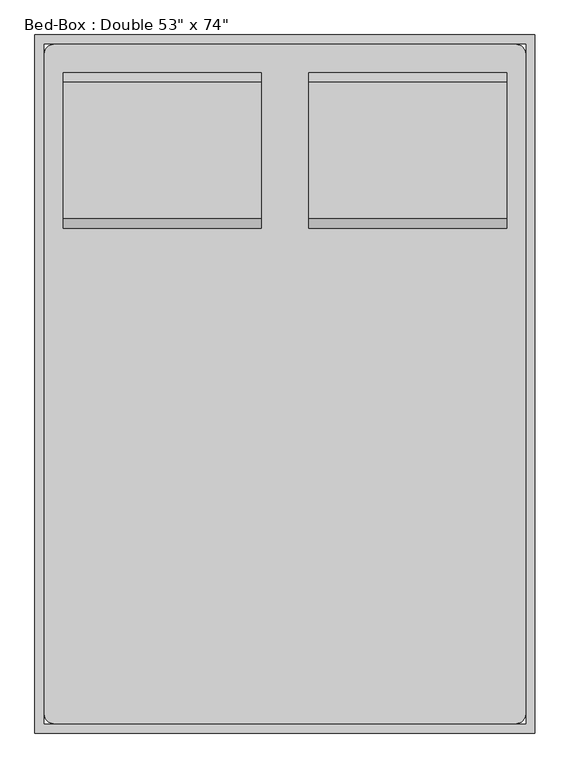
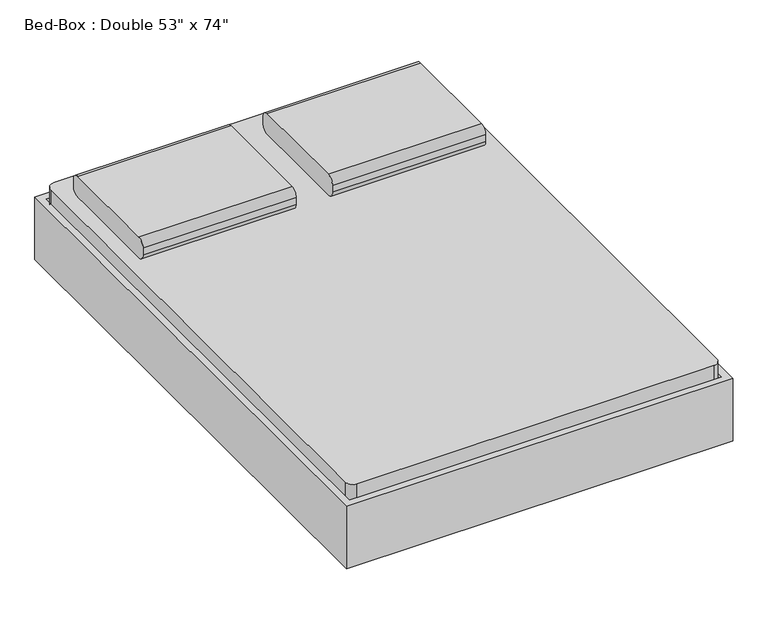
"""IFC4 building model written with IfcOpenShell, lengths in millimetres: furniture geometry."""

import ifcopenshell
import ifcopenshell.guid

model = None  # the IFC model being written
_history = None  # IfcOwnerHistory: only IFC2X3 demands one
_inside = {}  # id of a spatial element -> (the spatial element, [elements in it])
_under = {}  # id of a project, library or spatial element -> (it, [spatial elements below it])
_declared = {}  # id of a project -> (the project, [libraries it declares])
_typed = {}  # id of a type object -> (the type object, [elements of that type])
_made_of = {}  # id of a material, layer set ... -> (it, [elements and type objects made of it])


def new_model(schema):
    """Start an empty IFC model of exactly this schema.

    Asked for "IFC4X3", IfcOpenShell would pick the latest addendum, in which some entities
    have other attributes; the version numbers below select the first issue.
    IFC2X3 requires an IfcOwnerHistory on every rooted entity: one is made here for all.
    """
    global model, _history
    if schema == "IFC4X3":
        model = ifcopenshell.file(schema_version=(4, 3, 0, 0))
    else:
        model = ifcopenshell.file(schema=schema)
    _inside.clear()
    _under.clear()
    _declared.clear()
    _typed.clear()
    _made_of.clear()
    _history = None
    if model.schema == "IFC2X3":
        org = make("IfcOrganization", Name="unknown")
        user = make(
            "IfcPersonAndOrganization",
            ThePerson=make("IfcPerson", FamilyName="unknown"),
            TheOrganization=org,
        )
        app = make(
            "IfcApplication",
            ApplicationDeveloper=org,
            Version="unknown",
            ApplicationFullName="unknown",
            ApplicationIdentifier="unknown",
        )
        _history = make(
            "IfcOwnerHistory",
            OwningUser=user,
            OwningApplication=app,
            ChangeAction="ADDED",
            CreationDate=0,
        )
    return model


def make(cls, **values):
    """One entity of the class cls with the attributes given. An attribute that is None is left unset."""
    return model.create_entity(
        cls, **{name: value for name, value in values.items() if value is not None}
    )


def rooted(cls, **values):
    """An entity with a GlobalId (a new one), such as an element, a storey or a relation."""
    return make(cls, GlobalId=ifcopenshell.guid.new(), OwnerHistory=_history, **values)


def si_unit(unit_type, name, prefix=None):
    """IfcSIUnit, for example si_unit("LENGTHUNIT", "METRE", prefix="MILLI")."""
    return make("IfcSIUnit", UnitType=unit_type, Prefix=prefix, Name=name)


def assignment(units):
    """IfcUnitAssignment: the units of a project."""
    return None if units is None else make("IfcUnitAssignment", Units=units)


def point(xyz):
    """IfcCartesianPoint."""
    return None if xyz is None else make("IfcCartesianPoint", Coordinates=xyz)


def direction(xyz):
    """IfcDirection."""
    return None if xyz is None else make("IfcDirection", DirectionRatios=xyz)


def frame(location, z_axis=None, x_axis=None):
    """IfcAxis2Placement3D, a coordinate frame: its origin and axes. An axis left out is left unset."""
    return make(
        "IfcAxis2Placement3D",
        Location=point(location),
        Axis=direction(z_axis),
        RefDirection=direction(x_axis),
    )


def frame_2d(location, x_axis=None):
    """IfcAxis2Placement2D, a coordinate frame in the plane: its origin and x axis."""
    return make(
        "IfcAxis2Placement2D", Location=point(location), RefDirection=direction(x_axis)
    )


def origin():
    """The frame at (0, 0, 0) with its axes left unset."""
    return frame((0.0, 0.0, 0.0))


def place(relative_to, where):
    """IfcLocalPlacement: puts the frame where relative to a parent placement (None: the world)."""
    return make(
        "IfcLocalPlacement", PlacementRelTo=relative_to, RelativePlacement=where
    )


def context(
    kind, dimensions, precision=None, world=None, true_north=None, identifier=None
):
    """IfcGeometricRepresentationContext, for example the 3D "Model" context."""
    return make(
        "IfcGeometricRepresentationContext",
        ContextIdentifier=identifier,
        ContextType=kind,
        CoordinateSpaceDimension=dimensions,
        Precision=precision,
        WorldCoordinateSystem=world,
        TrueNorth=true_north,
    )


def project(units=None, contexts=None):
    """IfcProject with its units and contexts."""
    return rooted(
        "IfcProject",
        Name="project",
        RepresentationContexts=contexts,
        UnitsInContext=assignment(units),
    )


def spatial(cls, under=None, at=None, **own):
    """A site, building, storey or space (cls), placed at a placement, below another one or the project."""
    s = rooted(cls, ObjectPlacement=at, **own)
    if under is not None:
        _under.setdefault(under.id(), (under, []))[1].append(s)
    return s


def polyline(points):
    """IfcPolyline through the points."""
    return make("IfcPolyline", Points=[point(p) for p in points])


def circle_curve(where, radius):
    """IfcCircle in the frame where."""
    return make("IfcCircle", Position=where, Radius=radius)


def trimmed(basis, trim1, trim2, sense, master):
    """IfcTrimmedCurve: the piece of a basis curve between two trims."""
    return make(
        "IfcTrimmedCurve",
        BasisCurve=basis,
        Trim1=trim1,
        Trim2=trim2,
        SenseAgreement=sense,
        MasterRepresentation=master,
    )


def segment(curve, same_sense, transition):
    """IfcCompositeCurveSegment."""
    return make(
        "IfcCompositeCurveSegment",
        Transition=transition,
        SameSense=same_sense,
        ParentCurve=curve,
    )


def composite_curve(segments, self_intersect=None):
    """IfcCompositeCurve: segments joined end to end."""
    return make("IfcCompositeCurve", Segments=segments, SelfIntersect=self_intersect)


def outline(outer, holes=None, kind="AREA"):
    """IfcArbitraryClosedProfileDef: a profile drawn as a closed curve; with holes, ...WithVoids."""
    if holes is None:
        return make("IfcArbitraryClosedProfileDef", ProfileType=kind, OuterCurve=outer)
    return make(
        "IfcArbitraryProfileDefWithVoids",
        ProfileType=kind,
        OuterCurve=outer,
        InnerCurves=holes,
    )


def extrude(swept, where, along, depth):
    """IfcExtrudedAreaSolid: the profile swept, set in the frame where, extruded along a direction by depth."""
    return make(
        "IfcExtrudedAreaSolid",
        SweptArea=swept,
        Position=where,
        ExtrudedDirection=direction(along),
        Depth=depth,
    )


def shape(context_of_items, identifier, shape_type, items):
    """IfcShapeRepresentation: the items that make up one representation, for example the "Body"."""
    return make(
        "IfcShapeRepresentation",
        ContextOfItems=context_of_items,
        RepresentationIdentifier=identifier,
        RepresentationType=shape_type,
        Items=items,
    )


def source(mapping_origin, context_of_items, identifier, shape_type, items):
    """IfcRepresentationMap: a shape defined once, which mapped items show again and again."""
    return make(
        "IfcRepresentationMap",
        MappingOrigin=mapping_origin,
        MappedRepresentation=shape(context_of_items, identifier, shape_type, items),
    )


def transform(
    local_origin,
    x_axis=None,
    y_axis=None,
    z_axis=None,
    scale=None,
    scale2=None,
    scale3=None,
    uniform=True,
):
    """IfcCartesianTransformationOperator3D, or its non-uniform kind. x_axis, y_axis, z_axis: its Axis1, 2, 3."""
    if uniform:
        return make(
            "IfcCartesianTransformationOperator3D",
            Axis1=direction(x_axis),
            Axis2=direction(y_axis),
            LocalOrigin=point(local_origin),
            Scale=scale,
            Axis3=direction(z_axis),
        )
    return make(
        "IfcCartesianTransformationOperator3DnonUniform",
        Axis1=direction(x_axis),
        Axis2=direction(y_axis),
        LocalOrigin=point(local_origin),
        Scale=scale,
        Axis3=direction(z_axis),
        Scale2=scale2,
        Scale3=scale3,
    )


def mapped(mapping_source, mapping_target):
    """IfcMappedItem: shows the shape of a source again, moved by a transform."""
    return make(
        "IfcMappedItem", MappingSource=mapping_source, MappingTarget=mapping_target
    )


def made_of(thing, what):
    """Note that an element or type object is made of a material, layer set ...; save() writes the relation."""
    if what is not None:
        _made_of.setdefault(what.id(), (what, []))[1].append(thing)
    return thing


def element(
    cls,
    number,
    at=None,
    inside=None,
    cuts=None,
    type_object=None,
    material=None,
    context=None,
    identifier="Body",
    shape_type=None,
    held_by="IfcProductDefinitionShape",
    body=None,
    shapes=None,
    **own,
):
    """One element of the class cls, such as IfcWall. Its Tag is "e" and its number.

    at: its placement. inside: the storey or other place that contains it. cuts: it is an
    opening in that element (IfcRelVoidsElement). A single representation is given by context,
    identifier, shape_type and body (its items); several are given by shapes. held_by: the class
    of the entity that holds the representations. save() writes the other relations.
    """
    e = rooted(cls, Tag="e%d" % number, ObjectPlacement=at, **own)
    if body is not None:
        shapes = [shape(context, identifier, shape_type, body)]
    if shapes is not None:
        e.Representation = make(held_by, Representations=shapes)
    if inside is not None:
        _inside.setdefault(inside.id(), (inside, []))[1].append(e)
    if cuts is not None:
        rooted(
            "IfcRelVoidsElement", RelatingBuildingElement=cuts, RelatedOpeningElement=e
        )
    if type_object is not None:
        _typed.setdefault(type_object.id(), (type_object, []))[1].append(e)
    return made_of(e, material)


def aggregate(whole, parts):
    """IfcRelAggregates: a whole, such as a stair, and the parts it consists of."""
    return rooted("IfcRelAggregates", RelatingObject=whole, RelatedObjects=parts)


def save(model, path):
    """Write the relations noted so far, then the file.

    IfcRelAggregates (storeys below a building ...), IfcRelContainedInSpatialStructure (elements
    in a storey), IfcRelDefinesByType, IfcRelAssociatesMaterial and IfcRelDeclares: one each for
    every whole, place, type object, material and project.
    """
    for whole, parts in _under.values():
        aggregate(whole, parts)
    for where, things in _inside.values():
        rooted(
            "IfcRelContainedInSpatialStructure",
            RelatedElements=things,
            RelatingStructure=where,
        )
    for kind, things in _typed.values():
        rooted("IfcRelDefinesByType", RelatedObjects=things, RelatingType=kind)
    for what, things in _made_of.values():
        rooted("IfcRelAssociatesMaterial", RelatedObjects=things, RelatingMaterial=what)
    for by, libraries in _declared.values():
        rooted("IfcRelDeclares", RelatingContext=by, RelatedDefinitions=libraries)
    model.write(path)


def plane_surface(at):
    """IfcPlane: the flat surface through the origin of the frame at, square to its z axis."""
    return make("IfcPlane", Position=at)


def cylinder_surface(at, radius):
    """IfcCylindricalSurface: all points at the distance radius from the z axis of the frame at."""
    return make("IfcCylindricalSurface", Position=at, Radius=radius)


def revolved_surface(curve, axis_point, axis_direction):
    """IfcSurfaceOfRevolution: the curve turned about the line through axis_point along axis_direction."""
    return make(
        "IfcSurfaceOfRevolution",
        SweptCurve=make("IfcArbitraryOpenProfileDef", ProfileType="CURVE", Curve=curve),
        AxisPosition=make("IfcAxis1Placement", Location=point(axis_point), Axis=direction(axis_direction)),
    )


def advanced_brep(points, edges, surfaces, faces):
    """IfcAdvancedBrep: a solid bounded by faces that lie on surfaces and meet in shared edges.

    An edge is (start, end): straight between two places in points (the first is 0);
    or (start, end, curve); or (start, end, curve, False) where it runs against its curve.
    A face is (place in surfaces, loops), or (place, loops, False) where it looks against
    its surface's normal. A loop lists edges by number (the first is 1), with a minus sign
    where the edge is run from its end to its start. The first loop is the outer one.
    """
    corners = [point(p) for p in points]
    vertices = [make("IfcVertexPoint", VertexGeometry=c) for c in corners]
    made = []
    for start, end, *more in edges:
        made.append(
            make(
                "IfcEdgeCurve",
                EdgeStart=vertices[start],
                EdgeEnd=vertices[end],
                EdgeGeometry=more[0] if more else make("IfcPolyline", Points=[corners[start], corners[end]]),
                SameSense=more[1] if len(more) > 1 else True,
            )
        )
    hull = []
    for where, loops, *sense in faces:
        bounds = []
        for j, loop in enumerate(loops):
            ring = [make("IfcOrientedEdge", EdgeElement=made[abs(k) - 1], Orientation=k > 0) for k in loop]
            bounds.append(
                make(
                    "IfcFaceOuterBound" if j == 0 else "IfcFaceBound",
                    Bound=make("IfcEdgeLoop", EdgeList=ring),
                    Orientation=True,
                )
            )
        hull.append(make("IfcAdvancedFace", Bounds=bounds, FaceSurface=surfaces[where], SameSense=sense[0] if sense else True))
    return make("IfcAdvancedBrep", Outer=make("IfcClosedShell", CfsFaces=hull))


def furniture_bd6c971a(model_context):
    return source(origin(), model_context, "Body", "SolidModel", [
        extrude(outline(composite_curve([segment(polyline([(578.3704918, 406.4), (210.0704918, 406.4)]), True, "CONTINUOUS"), segment(trimmed(circle_curve(frame_2d((210.0704918, 431.8)), 25.4), [point((210.0704918, 406.4))], [point((184.6704918, 431.8))], False, "CARTESIAN"), True, "CONTINUOUS"), segment(polyline([(184.6704918, 431.8), (184.6704918, 457.2)]), True, "CONTINUOUS"), segment(trimmed(circle_curve(frame_2d((210.0704918, 457.2)), 25.4), [point((184.6704918, 457.2))], [point((210.0704918, 482.6))], False, "CARTESIAN"), True, "CONTINUOUS"), segment(polyline([(210.0704918, 482.6), (578.3704918, 482.6)]), True, "CONTINUOUS"), segment(trimmed(circle_curve(frame_2d((578.3704918, 457.2)), 25.4), [point((578.3704918, 482.6))], [point((603.7704918, 457.2))], False, "CARTESIAN"), True, "CONTINUOUS"), segment(polyline([(603.7704918, 457.2), (603.7704918, 431.8)]), True, "CONTINUOUS"), segment(trimmed(circle_curve(frame_2d((578.3704918, 431.8)), 25.4), [point((603.7704918, 431.8))], [point((578.3704918, 406.4))], False, "CARTESIAN"), True, "CONTINUOUS")], self_intersect=False)), frame((402.652459, 0.0, 0.0), z_axis=(1.0, 0.0, 0.0), x_axis=(0.0, 1.0, 0.0)), (0.0, 0.0, 1.0), 533.4),
        extrude(outline(composite_curve([segment(polyline([(578.3704918, 406.4), (210.0704918, 406.4)]), True, "CONTINUOUS"), segment(trimmed(circle_curve(frame_2d((210.0704918, 431.8)), 25.4), [point((210.0704918, 406.4))], [point((184.6704918, 431.8))], False, "CARTESIAN"), True, "CONTINUOUS"), segment(polyline([(184.6704918, 431.8), (184.6704918, 457.2)]), True, "CONTINUOUS"), segment(trimmed(circle_curve(frame_2d((210.0704918, 457.2)), 25.4), [point((184.6704918, 457.2))], [point((210.0704918, 482.6))], False, "CARTESIAN"), True, "CONTINUOUS"), segment(polyline([(210.0704918, 482.6), (578.3704918, 482.6)]), True, "CONTINUOUS"), segment(trimmed(circle_curve(frame_2d((578.3704918, 457.2)), 25.4), [point((578.3704918, 482.6))], [point((603.7704918, 457.2))], False, "CARTESIAN"), True, "CONTINUOUS"), segment(polyline([(603.7704918, 457.2), (603.7704918, 431.8)]), True, "CONTINUOUS"), segment(trimmed(circle_curve(frame_2d((578.3704918, 431.8)), 25.4), [point((603.7704918, 431.8))], [point((578.3704918, 406.4))], False, "CARTESIAN"), True, "CONTINUOUS")], self_intersect=False)), frame((-257.747541, 0.0, 0.0), z_axis=(1.0, 0.0, 0.0), x_axis=(0.0, 1.0, 0.0)), (0.0, 0.0, 1.0), 533.4),
        advanced_brep(
        [(-308.2231784, 451.3704918, 177.8), (-308.2231784, 375.1704918, 177.8), (-308.2231784, 375.1704918, 196.85), (-308.2231784, 451.3704918, 196.85), (-257.4231784, 451.3704918, 177.8), (-257.4231784, 375.1704918, 177.8), (-245.2869899, 375.1704918, 196.85), (-245.2869899, 451.3704918, 196.85), (-181.3523099, 451.3704918, 14.6654962), (-181.3523099, 375.1704918, 14.6654962), (-164.0871466, 375.1704918, 22.716374), (-164.0871466, 451.3704918, 22.716374), (-158.3320921, 375.1704918, 0.0), (-158.3320921, 451.3704918, 0.0), (-158.3320921, 375.1704918, 19.05), (-158.3320921, 451.3704918, 19.05), (-79.7195862, 451.3704918, 0.0), (-79.7195862, 375.1704918, 0.0), (-79.7195862, 375.1704918, 19.05), (-79.7195862, 451.3704918, 19.05), (-67.0195862, 375.1704918, 3.4029547), (-67.0195862, 451.3704918, 3.4029547), (-76.5445862, 375.1704918, 19.9007387), (-76.5445862, 451.3704918, 19.9007387), (-6.922541, 451.3704918, 38.1), (-6.922541, 375.1704918, 38.1), (-12.0269731, 375.1704918, 57.15), (-12.0269731, 451.3704918, 57.15), (685.5518216, 451.3704918, 38.1), (685.5518216, 375.1704918, 38.1), (690.6562537, 375.1704918, 57.15), (690.6562537, 451.3704918, 57.15), (745.6488669, 451.3704918, 3.4029547), (745.6488669, 375.1704918, 3.4029547), (755.1738669, 375.1704918, 19.9007387), (755.1738669, 451.3704918, 19.9007387), (758.3488669, 375.1704918, 0.0), (758.3488669, 451.3704918, 0.0), (758.3488669, 375.1704918, 19.05), (758.3488669, 451.3704918, 19.05), (836.9613728, 451.3704918, 0.0), (836.9613728, 375.1704918, 0.0), (836.9613728, 375.1704918, 19.05), (836.9613728, 451.3704918, 19.05), (859.9815906, 375.1704918, 14.6654962), (859.9815906, 451.3704918, 14.6654962), (842.7164272, 375.1704918, 22.716374), (842.7164272, 451.3704918, 22.716374), (936.052459, 451.3704918, 177.8), (936.052459, 375.1704918, 177.8), (923.9162705, 375.1704918, 196.85), (923.9162705, 451.3704918, 196.85), (986.852459, 451.3704918, 177.8), (986.852459, 451.3704918, 196.85), (986.852459, 375.1704918, 196.85), (986.852459, 375.1704918, 177.8)],
        [
            (0, 1),
            (1, 2),
            (2, 3),
            (3, 0),
            (0, 4),
            (4, 5),
            (5, 1),
            (5, 6),
            (6, 2),
            (6, 7),
            (7, 3),
            (7, 4),
            (4, 8),
            (8, 9),
            (9, 5),
            (9, 10),
            (10, 6),
            (10, 11),
            (11, 7),
            (11, 8),
            (12, 9, circle_curve(frame((-158.3320921, 375.1704918, 25.4), z_axis=(0.0, 1.0, 0.0), x_axis=(-0.9063077870366486, 0.0, -0.42261826174070233)), 25.4)),
            (8, 13, circle_curve(frame((-158.3320921, 451.3704918, 25.4), z_axis=(0.0, -1.0, 0.0), x_axis=(-0.9063077870366486, 0.0, -0.42261826174070233)), 25.4)),
            (13, 12),
            (14, 10, circle_curve(frame((-158.3320921, 375.1704918, 25.4), z_axis=(0.0, 1.0, 0.0), x_axis=(-0.9063077870366486, 0.0, -0.42261826174070233)), 6.35)),
            (12, 14),
            (15, 11, circle_curve(frame((-158.3320921, 451.3704918, 25.4), z_axis=(0.0, 1.0, 0.0), x_axis=(-0.9063077870366486, 0.0, -0.42261826174070233)), 6.35)),
            (14, 15),
            (15, 13),
            (13, 16),
            (16, 17),
            (17, 12),
            (17, 18),
            (18, 14),
            (18, 19),
            (19, 15),
            (19, 16),
            (20, 17, circle_curve(frame((-79.7195862, 375.1704918, 25.4), z_axis=(0.0, 1.0, 0.0), x_axis=(0.0, 0.0, -1.0)), 25.4)),
            (16, 21, circle_curve(frame((-79.7195862, 451.3704918, 25.4), z_axis=(0.0, -1.0, 0.0), x_axis=(0.0, 0.0, -1.0)), 25.4)),
            (21, 20),
            (22, 18, circle_curve(frame((-79.7195862, 375.1704918, 25.4), z_axis=(0.0, 1.0, 0.0), x_axis=(0.0, 0.0, -1.0)), 6.35)),
            (20, 22),
            (23, 19, circle_curve(frame((-79.7195862, 451.3704918, 25.4), z_axis=(0.0, 1.0, 0.0), x_axis=(0.0, 0.0, -1.0)), 6.35)),
            (22, 23),
            (23, 21),
            (21, 24),
            (24, 25),
            (25, 20),
            (25, 26),
            (26, 22),
            (26, 27),
            (27, 23),
            (27, 24),
            (24, 28),
            (28, 29),
            (29, 25),
            (29, 30),
            (30, 26),
            (30, 31),
            (31, 27),
            (31, 28),
            (28, 32),
            (32, 33),
            (33, 29),
            (33, 34),
            (34, 30),
            (34, 35),
            (35, 31),
            (35, 32),
            (36, 33, circle_curve(frame((758.3488669, 375.1704918, 25.4), z_axis=(0.0, 1.0, 0.0), x_axis=(-0.5000000000000463, 0.0, -0.8660254037844118)), 25.4)),
            (32, 37, circle_curve(frame((758.3488669, 451.3704918, 25.4), z_axis=(0.0, -1.0, 0.0), x_axis=(-0.5000000000000463, 0.0, -0.8660254037844118)), 25.4)),
            (37, 36),
            (38, 34, circle_curve(frame((758.3488669, 375.1704918, 25.4), z_axis=(0.0, 1.0, 0.0), x_axis=(-0.5000000000000463, 0.0, -0.8660254037844118)), 6.35)),
            (36, 38),
            (39, 35, circle_curve(frame((758.3488669, 451.3704918, 25.4), z_axis=(0.0, 1.0, 0.0), x_axis=(-0.5000000000000463, 0.0, -0.8660254037844118)), 6.35)),
            (38, 39),
            (39, 37),
            (37, 40),
            (40, 41),
            (41, 36),
            (41, 42),
            (42, 38),
            (42, 43),
            (43, 39),
            (43, 40),
            (44, 41, circle_curve(frame((836.9613728, 375.1704918, 25.4), z_axis=(0.0, 1.0, 0.0), x_axis=(0.0, 0.0, -1.0)), 25.4)),
            (40, 45, circle_curve(frame((836.9613728, 451.3704918, 25.4), z_axis=(0.0, -1.0, 0.0), x_axis=(0.0, 0.0, -1.0)), 25.4)),
            (45, 44),
            (46, 42, circle_curve(frame((836.9613728, 375.1704918, 25.4), z_axis=(0.0, 1.0, 0.0), x_axis=(0.0, 0.0, -1.0)), 6.35)),
            (44, 46),
            (47, 43, circle_curve(frame((836.9613728, 451.3704918, 25.4), z_axis=(0.0, 1.0, 0.0), x_axis=(0.0, 0.0, -1.0)), 6.35)),
            (46, 47),
            (47, 45),
            (45, 48),
            (48, 49),
            (49, 44),
            (49, 50),
            (50, 46),
            (50, 51),
            (51, 47),
            (51, 48),
            (52, 53),
            (53, 54),
            (54, 55),
            (55, 52),
            (48, 52),
            (55, 49),
            (54, 50),
            (53, 51),
        ],
        [
            plane_surface(frame((-308.2231784, 705.3704918, -152.9490627), z_axis=(-1.0, 0.0, 0.0), x_axis=(0.0, 1.0, 0.0))),
            plane_surface(frame((-308.2231784, 451.3704918, 177.8), z_axis=(0.0, 0.0, -1.0), x_axis=(1.0, 0.0, 0.0))),
            plane_surface(frame((-308.2231784, 375.1704918, 177.8), z_axis=(0.0, -1.0, 0.0), x_axis=(1.0, 0.0, 0.0))),
            plane_surface(frame((-308.2231784, 375.1704918, 196.85), z_axis=(0.0, 0.0, 1.0), x_axis=(1.0, 0.0, 0.0))),
            plane_surface(frame((-308.2231784, 451.3704918, 196.85), z_axis=(0.0, 1.0, 0.0), x_axis=(1.0, 0.0, 0.0))),
            plane_surface(frame((-257.4231784, 451.3704918, 177.8), z_axis=(-0.9063077870366488, 0.0, -0.42261826174070194), x_axis=(0.42261826174070194, 0.0, -0.9063077870366488))),
            plane_surface(frame((-257.4231784, 375.1704918, 177.8), z_axis=(0.0, -1.0, 0.0), x_axis=(0.42261826174070194, 0.0, -0.9063077870366488))),
            plane_surface(frame((-245.2869899, 375.1704918, 196.85), z_axis=(0.9063077870366487, 0.0, 0.4226182617407021), x_axis=(0.4226182617407021, 0.0, -0.9063077870366487))),
            plane_surface(frame((-245.2869899, 451.3704918, 196.85), z_axis=(0.0, 1.0, 0.0), x_axis=(0.4226182617407021, 0.0, -0.9063077870366487))),
            cylinder_surface(frame((-158.3320921, 705.3704918, 25.4), z_axis=(0.0, -1.0, 0.0), x_axis=(-0.9063077870366486, 0.0, -0.42261826174070233)), 25.4),
            plane_surface(frame((-158.3320921, 375.1704918, 25.4), z_axis=(0.0, -1.0, 0.0), x_axis=(-0.9063077870366486, 0.0, -0.42261826174070233))),
            revolved_surface(polyline([(-164.08714654768272, 375.1704918, 22.71637403794654), (-164.08714654768272, 451.3704918, 22.71637403794654)]), (-158.3320921, 705.3704918, 25.4), (0.0, -1.0, 0.0)),
            plane_surface(frame((-158.3320921, 451.3704918, 25.4), z_axis=(0.0, 1.0, 0.0), x_axis=(-0.9063077870366486, 0.0, -0.42261826174070233))),
            plane_surface(frame((-158.3320921, 451.3704918, 0.0), z_axis=(0.0, 0.0, -1.0), x_axis=(1.0, 0.0, 0.0))),
            plane_surface(frame((-158.3320921, 375.1704918, 0.0), z_axis=(0.0, -1.0, 0.0), x_axis=(1.0, 0.0, 0.0))),
            plane_surface(frame((-158.3320921, 375.1704918, 19.05), z_axis=(0.0, 0.0, 1.0), x_axis=(1.0, 0.0, 0.0))),
            plane_surface(frame((-158.3320921, 451.3704918, 19.05), z_axis=(0.0, 1.0, 0.0), x_axis=(1.0, 0.0, 0.0))),
            cylinder_surface(frame((-79.7195862, 705.3704918, 25.4), z_axis=(0.0, -1.0, 0.0), x_axis=(0.0, 0.0, -1.0)), 25.4),
            plane_surface(frame((-79.7195862, 375.1704918, 25.4), z_axis=(0.0, -1.0, 0.0), x_axis=(0.0, 0.0, -1.0))),
            revolved_surface(polyline([(-79.7195862, 375.1704918, 19.049999999999997), (-79.7195862, 451.3704918, 19.049999999999997)]), (-79.7195862, 705.3704918, 25.4), (0.0, -1.0, 0.0)),
            plane_surface(frame((-79.7195862, 451.3704918, 25.4), z_axis=(0.0, 1.0, 0.0), x_axis=(0.0, 0.0, -1.0))),
            plane_surface(frame((-67.0195862, 451.3704918, 3.4029547), z_axis=(0.4999999999998774, 0.0, -0.8660254037845095), x_axis=(0.8660254037845095, 0.0, 0.4999999999998774))),
            plane_surface(frame((-67.0195862, 375.1704918, 3.4029547), z_axis=(0.0, -1.0, 0.0), x_axis=(0.866025403784509, 0.0, 0.49999999999987815))),
            plane_surface(frame((-76.5445862, 375.1704918, 19.9007387), z_axis=(-0.49999999999987754, 0.0, 0.8660254037845093), x_axis=(0.8660254037845093, 0.0, 0.49999999999987754))),
            plane_surface(frame((-76.5445862, 451.3704918, 19.9007387), z_axis=(0.0, 1.0000000000000002, 0.0), x_axis=(0.8660254037845091, 0.0, 0.49999999999987815))),
            plane_surface(frame((-6.922541, 451.3704918, 38.1), z_axis=(0.0, 0.0, -1.0), x_axis=(1.0, 0.0, 0.0))),
            plane_surface(frame((-6.922541, 375.1704918, 38.1), z_axis=(0.0, -1.0, 0.0), x_axis=(1.0, 0.0, 0.0))),
            plane_surface(frame((-12.0269731, 375.1704918, 57.15), z_axis=(0.0, 0.0, 1.0), x_axis=(1.0, 0.0, 0.0))),
            plane_surface(frame((-12.0269731, 451.3704918, 57.15), z_axis=(0.0, 1.0, 0.0), x_axis=(1.0, 0.0, 0.0))),
            plane_surface(frame((685.5518216, 451.3704918, 38.1), z_axis=(-0.500000000000047, 0.0, -0.8660254037844115), x_axis=(0.8660254037844115, 0.0, -0.500000000000047))),
            plane_surface(frame((685.5518216, 375.1704918, 38.1), z_axis=(0.0, -1.0, 0.0), x_axis=(0.8660254037844116, 0.0, -0.500000000000047))),
            plane_surface(frame((690.6562537, 375.1704918, 57.15), z_axis=(0.5000000000000456, 0.0, 0.8660254037844124), x_axis=(0.8660254037844124, 0.0, -0.5000000000000456))),
            plane_surface(frame((690.6562537, 451.3704918, 57.15), z_axis=(0.0, 1.0, 0.0), x_axis=(0.8660254037844124, 0.0, -0.5000000000000456))),
            cylinder_surface(frame((758.3488669, 705.3704918, 25.4), z_axis=(0.0, -1.0, 0.0), x_axis=(-0.5000000000000463, 0.0, -0.8660254037844118)), 25.4),
            plane_surface(frame((758.3488669, 375.1704918, 25.4), z_axis=(0.0, -1.0000000000000002, 0.0), x_axis=(-0.5000000000000464, 0.0, -0.866025403784412))),
            revolved_surface(polyline([(755.1738668999997, 375.1704918, 19.90073868596898), (755.1738668999997, 451.3704918, 19.90073868596898)]), (758.3488669, 705.3704918, 25.4), (0.0, -1.0, 0.0)),
            plane_surface(frame((758.3488669, 451.3704918, 25.4), z_axis=(0.0, 1.0000000000000002, 0.0), x_axis=(-0.5000000000000464, 0.0, -0.866025403784412))),
            plane_surface(frame((758.3488669, 451.3704918, 0.0), z_axis=(0.0, 0.0, -1.0), x_axis=(1.0, 0.0, 0.0))),
            plane_surface(frame((758.3488669, 375.1704918, 0.0), z_axis=(0.0, -1.0, 0.0), x_axis=(1.0, 0.0, 0.0))),
            plane_surface(frame((758.3488669, 375.1704918, 19.05), z_axis=(0.0, 0.0, 1.0), x_axis=(1.0, 0.0, 0.0))),
            plane_surface(frame((758.3488669, 451.3704918, 19.05), z_axis=(0.0, 1.0, 0.0), x_axis=(1.0, 0.0, 0.0))),
            cylinder_surface(frame((836.9613728, 705.3704918, 25.4), z_axis=(0.0, -1.0, 0.0), x_axis=(0.0, 0.0, -1.0)), 25.4),
            plane_surface(frame((836.9613728, 375.1704918, 25.4), z_axis=(0.0, -1.0, 0.0), x_axis=(0.0, 0.0, -1.0))),
            revolved_surface(polyline([(836.9613728, 375.1704918, 19.049999999999997), (836.9613728, 451.3704918, 19.049999999999997)]), (836.9613728, 705.3704918, 25.4), (0.0, -1.0, 0.0)),
            plane_surface(frame((836.9613728, 451.3704918, 25.4), z_axis=(0.0, 1.0, 0.0), x_axis=(0.0, 0.0, -1.0))),
            plane_surface(frame((859.9815906, 451.3704918, 14.6654962), z_axis=(0.9063077870366798, 0.0, -0.4226182617406355), x_axis=(0.4226182617406355, 0.0, 0.9063077870366798))),
            plane_surface(frame((859.9815906, 375.1704918, 14.6654962), z_axis=(0.0, -1.0, 0.0), x_axis=(0.4226182617406356, 0.0, 0.9063077870366797))),
            plane_surface(frame((842.7164272, 375.1704918, 22.716374), z_axis=(-0.9063077870366797, 0.0, 0.4226182617406358), x_axis=(0.4226182617406358, 0.0, 0.9063077870366797))),
            plane_surface(frame((842.7164272, 451.3704918, 22.716374), z_axis=(0.0, 1.0000000000000002, 0.0), x_axis=(0.42261826174063544, 0.0, 0.9063077870366799))),
            plane_surface(frame((986.852459, 705.3704918, -152.9490627), z_axis=(1.0, 0.0, 0.0), x_axis=(0.0, 1.0, 0.0))),
            plane_surface(frame((936.052459, 451.3704918, 177.8), z_axis=(0.0, 0.0, -1.0), x_axis=(1.0, 0.0, 0.0))),
            plane_surface(frame((936.052459, 375.1704918, 177.8), z_axis=(0.0, -1.0, 0.0), x_axis=(1.0, 0.0, 0.0))),
            plane_surface(frame((923.9162705, 375.1704918, 196.85), z_axis=(0.0, 0.0, 1.0), x_axis=(1.0, 0.0, 0.0))),
            plane_surface(frame((923.9162705, 451.3704918, 196.85), z_axis=(0.0, 1.0, 0.0), x_axis=(1.0, 0.0, 0.0))),
        ],
        [
            (0, [[1, 2, 3, 4]]),
            (1, [[-1, 5, 6, 7]]),
            (2, [[-2, -7, 8, 9]]),
            (3, [[-3, -9, 10, 11]]),
            (4, [[-4, -11, 12, -5]]),
            (5, [[-6, 13, 14, 15]]),
            (6, [[-8, -15, 16, 17]]),
            (7, [[-10, -17, 18, 19]]),
            (8, [[-12, -19, 20, -13]]),
            (9, [[21, -14, 22, 23]]),
            (10, [[24, -16, -21, 25]]),
            (11, [[26, -18, -24, 27]]),
            (12, [[-22, -20, -26, 28]]),
            (13, [[-23, 29, 30, 31]]),
            (14, [[-25, -31, 32, 33]]),
            (15, [[-27, -33, 34, 35]]),
            (16, [[-28, -35, 36, -29]]),
            (17, [[37, -30, 38, 39]]),
            (18, [[40, -32, -37, 41]]),
            (19, [[42, -34, -40, 43]]),
            (20, [[-38, -36, -42, 44]]),
            (21, [[-39, 45, 46, 47]]),
            (22, [[-41, -47, 48, 49]]),
            (23, [[-43, -49, 50, 51]]),
            (24, [[-44, -51, 52, -45]]),
            (25, [[-46, 53, 54, 55]]),
            (26, [[-48, -55, 56, 57]]),
            (27, [[-50, -57, 58, 59]]),
            (28, [[-52, -59, 60, -53]]),
            (29, [[-54, 61, 62, 63]]),
            (30, [[-56, -63, 64, 65]]),
            (31, [[-58, -65, 66, 67]]),
            (32, [[-60, -67, 68, -61]]),
            (33, [[69, -62, 70, 71]]),
            (34, [[72, -64, -69, 73]]),
            (35, [[74, -66, -72, 75]]),
            (36, [[-70, -68, -74, 76]]),
            (37, [[-71, 77, 78, 79]]),
            (38, [[-73, -79, 80, 81]]),
            (39, [[-75, -81, 82, 83]]),
            (40, [[-76, -83, 84, -77]]),
            (41, [[85, -78, 86, 87]]),
            (42, [[88, -80, -85, 89]]),
            (43, [[90, -82, -88, 91]]),
            (44, [[-86, -84, -90, 92]]),
            (45, [[-87, 93, 94, 95]]),
            (46, [[-89, -95, 96, 97]]),
            (47, [[-91, -97, 98, 99]]),
            (48, [[-92, -99, 100, -93]]),
            (49, [[101, 102, 103, 104]]),
            (50, [[-94, 105, -104, 106]]),
            (51, [[-96, -106, -103, 107]]),
            (52, [[-98, -107, -102, 108]]),
            (53, [[-100, -108, -101, -105]]),
        ],
    ),
        extrude(outline(composite_curve([segment(polyline([(-283.147541, 679.9704918), (961.452459, 679.9704918)]), True, "CONTINUOUS"), segment(trimmed(circle_curve(frame_2d((961.452459, 654.5704918)), 25.4), [point((961.452459, 679.9704918))], [point((986.852459, 654.5704918))], False, "CARTESIAN"), True, "CONTINUOUS"), segment(polyline([(986.852459, 654.5704918), (986.852459, -1123.4295082)]), True, "CONTINUOUS"), segment(trimmed(circle_curve(frame_2d((961.452459, -1123.4295082)), 25.4), [point((986.852459, -1123.4295082))], [point((961.452459, -1148.8295082))], False, "CARTESIAN"), True, "CONTINUOUS"), segment(polyline([(961.452459, -1148.8295082), (-283.147541, -1148.8295082)]), True, "CONTINUOUS"), segment(trimmed(circle_curve(frame_2d((-283.147541, -1123.4295082)), 25.4), [point((-283.147541, -1148.8295082))], [point((-308.547541, -1123.4295082))], False, "CARTESIAN"), True, "CONTINUOUS"), segment(polyline([(-308.547541, -1123.4295082), (-308.547541, 654.5704918)]), True, "CONTINUOUS"), segment(trimmed(circle_curve(frame_2d((-283.147541, 654.5704918)), 25.4), [point((-308.547541, 654.5704918))], [point((-283.147541, 679.9704918))], False, "CARTESIAN"), True, "CONTINUOUS")], self_intersect=False)), frame((0.0, 0.0, 203.2), z_axis=(0.0, 0.0, 1.0), x_axis=(1.0, 0.0, 0.0)), (0.0, 0.0, 1.0), 203.2),
        advanced_brep(
        [(-308.547541, -869.4295082, 196.85), (-308.547541, -869.4295082, 177.8), (-308.547541, -945.6295082, 177.8), (-308.547541, -945.6295082, 196.85), (-245.6113525, -869.4295082, 196.85), (-257.747541, -869.4295082, 177.8), (-257.747541, -945.6295082, 177.8), (-245.6113525, -945.6295082, 196.85), (-164.4115092, -869.4295082, 22.716374), (-181.6766725, -869.4295082, 14.6654962), (-181.6766725, -945.6295082, 14.6654962), (-164.4115092, -945.6295082, 22.716374), (-158.6564547, -869.4295082, 0.0), (-158.6564547, -869.4295082, 19.05), (-158.6564547, -945.6295082, 0.0), (-158.6564547, -945.6295082, 19.05), (-80.0439489, -869.4295082, 19.05), (-80.0439489, -869.4295082, 0.0), (-80.0439489, -945.6295082, 0.0), (-80.0439489, -945.6295082, 19.05), (-67.3439489, -869.4295082, 3.4029547), (-76.8689489, -869.4295082, 19.9007387), (-67.3439489, -945.6295082, 3.4029547), (-76.8689489, -945.6295082, 19.9007387), (-12.3513357, -869.4295082, 57.15), (-7.2469036, -869.4295082, 38.1), (-7.2469036, -945.6295082, 38.1), (-12.3513357, -945.6295082, 57.15), (690.6562537, -869.4295082, 57.15), (685.5518216, -869.4295082, 38.1), (685.5518216, -945.6295082, 38.1), (690.6562537, -945.6295082, 57.15), (755.1738669, -869.4295082, 19.9007387), (745.6488669, -869.4295082, 3.4029547), (745.6488669, -945.6295082, 3.4029547), (755.1738669, -945.6295082, 19.9007387), (758.3488669, -869.4295082, 0.0), (758.3488669, -869.4295082, 19.05), (758.3488669, -945.6295082, 0.0), (758.3488669, -945.6295082, 19.05), (836.9613728, -869.4295082, 19.05), (836.9613728, -869.4295082, 0.0), (836.9613728, -945.6295082, 0.0), (836.9613728, -945.6295082, 19.05), (859.9815906, -869.4295082, 14.6654962), (842.7164272, -869.4295082, 22.716374), (859.9815906, -945.6295082, 14.6654962), (842.7164272, -945.6295082, 22.716374), (923.9162705, -869.4295082, 196.85), (936.052459, -869.4295082, 177.8), (936.052459, -945.6295082, 177.8), (923.9162705, -945.6295082, 196.85), (986.852459, -869.4295082, 196.85), (986.852459, -945.6295082, 196.85), (986.852459, -945.6295082, 177.8), (986.852459, -869.4295082, 177.8)],
        [
            (0, 1),
            (1, 2),
            (2, 3),
            (3, 0),
            (0, 4),
            (4, 5),
            (5, 1),
            (5, 6),
            (6, 2),
            (6, 7),
            (7, 3),
            (7, 4),
            (4, 8),
            (8, 9),
            (9, 5),
            (9, 10),
            (10, 6),
            (10, 11),
            (11, 7),
            (11, 8),
            (12, 9, circle_curve(frame((-158.6564547, -869.4295082, 25.4), z_axis=(0.0, 1.0, 0.0), x_axis=(-0.906307787036663, 0.0, -0.4226182617406713)), 25.4)),
            (8, 13, circle_curve(frame((-158.6564547, -869.4295082, 25.4), z_axis=(0.0, -1.0, 0.0), x_axis=(-0.906307787036663, 0.0, -0.4226182617406713)), 6.35)),
            (13, 12),
            (14, 10, circle_curve(frame((-158.6564547, -945.6295082, 25.4), z_axis=(0.0, 1.0, 0.0), x_axis=(-0.906307787036663, 0.0, -0.4226182617406713)), 25.4)),
            (12, 14),
            (15, 11, circle_curve(frame((-158.6564547, -945.6295082, 25.4), z_axis=(0.0, 1.0, 0.0), x_axis=(-0.906307787036663, 0.0, -0.4226182617406713)), 6.35)),
            (14, 15),
            (15, 13),
            (13, 16),
            (16, 17),
            (17, 12),
            (17, 18),
            (18, 14),
            (18, 19),
            (19, 15),
            (19, 16),
            (20, 17, circle_curve(frame((-80.0439489, -869.4295082, 25.4), z_axis=(0.0, 1.0, 0.0), x_axis=(0.0, 0.0, -1.0)), 25.4)),
            (16, 21, circle_curve(frame((-80.0439489, -869.4295082, 25.4), z_axis=(0.0, -1.0, 0.0), x_axis=(0.0, 0.0, -1.0)), 6.35)),
            (21, 20),
            (22, 18, circle_curve(frame((-80.0439489, -945.6295082, 25.4), z_axis=(0.0, 1.0, 0.0), x_axis=(0.0, 0.0, -1.0)), 25.4)),
            (20, 22),
            (23, 19, circle_curve(frame((-80.0439489, -945.6295082, 25.4), z_axis=(0.0, 1.0, 0.0), x_axis=(0.0, 0.0, -1.0)), 6.35)),
            (22, 23),
            (23, 21),
            (21, 24),
            (24, 25),
            (25, 20),
            (25, 26),
            (26, 22),
            (26, 27),
            (27, 23),
            (27, 24),
            (24, 28),
            (28, 29),
            (29, 25),
            (29, 30),
            (30, 26),
            (30, 31),
            (31, 27),
            (31, 28),
            (28, 32),
            (32, 33),
            (33, 29),
            (33, 34),
            (34, 30),
            (34, 35),
            (35, 31),
            (35, 32),
            (36, 33, circle_curve(frame((758.3488669, -869.4295082, 25.4), z_axis=(0.0, 1.0, 0.0), x_axis=(-0.5000000000000479, 0.0, -0.866025403784411)), 25.4)),
            (32, 37, circle_curve(frame((758.3488669, -869.4295082, 25.4), z_axis=(0.0, -1.0, 0.0), x_axis=(-0.5000000000000479, 0.0, -0.866025403784411)), 6.35)),
            (37, 36),
            (38, 34, circle_curve(frame((758.3488669, -945.6295082, 25.4), z_axis=(0.0, 1.0, 0.0), x_axis=(-0.5000000000000479, 0.0, -0.866025403784411)), 25.4)),
            (36, 38),
            (39, 35, circle_curve(frame((758.3488669, -945.6295082, 25.4), z_axis=(0.0, 1.0, 0.0), x_axis=(-0.5000000000000479, 0.0, -0.866025403784411)), 6.35)),
            (38, 39),
            (39, 37),
            (37, 40),
            (40, 41),
            (41, 36),
            (41, 42),
            (42, 38),
            (42, 43),
            (43, 39),
            (43, 40),
            (44, 41, circle_curve(frame((836.9613728, -869.4295082, 25.4), z_axis=(0.0, 1.0, 0.0), x_axis=(0.0, 0.0, -1.0)), 25.4)),
            (40, 45, circle_curve(frame((836.9613728, -869.4295082, 25.4), z_axis=(0.0, -1.0, 0.0), x_axis=(0.0, 0.0, -1.0)), 6.35)),
            (45, 44),
            (46, 42, circle_curve(frame((836.9613728, -945.6295082, 25.4), z_axis=(0.0, 1.0, 0.0), x_axis=(0.0, 0.0, -1.0)), 25.4)),
            (44, 46),
            (47, 43, circle_curve(frame((836.9613728, -945.6295082, 25.4), z_axis=(0.0, 1.0, 0.0), x_axis=(0.0, 0.0, -1.0)), 6.35)),
            (46, 47),
            (47, 45),
            (45, 48),
            (48, 49),
            (49, 44),
            (49, 50),
            (50, 46),
            (50, 51),
            (51, 47),
            (51, 48),
            (52, 53),
            (53, 54),
            (54, 55),
            (55, 52),
            (48, 52),
            (55, 49),
            (54, 50),
            (53, 51),
        ],
        [
            plane_surface(frame((-308.547541, -1174.2295082, -127.5947323), z_axis=(-1.0, 0.0, 0.0), x_axis=(0.0, 1.0, 0.0))),
            plane_surface(frame((-308.547541, -869.4295082, 196.85), z_axis=(0.0, 1.0, 0.0), x_axis=(1.0, 0.0, 0.0))),
            plane_surface(frame((-308.547541, -869.4295082, 177.8), z_axis=(0.0, 0.0, -1.0), x_axis=(1.0, 0.0, 0.0))),
            plane_surface(frame((-308.547541, -945.6295082, 177.8), z_axis=(0.0, -1.0, 0.0), x_axis=(1.0, 0.0, 0.0))),
            plane_surface(frame((-308.547541, -945.6295082, 196.85), z_axis=(0.0, 0.0, 1.0), x_axis=(1.0, 0.0, 0.0))),
            plane_surface(frame((-245.6113525, -869.4295082, 196.85), z_axis=(0.0, 1.0, 0.0), x_axis=(0.422618261740671, 0.0, -0.9063077870366633))),
            plane_surface(frame((-257.747541, -869.4295082, 177.8), z_axis=(-0.9063077870366631, 0.0, -0.42261826174067113), x_axis=(0.42261826174067113, 0.0, -0.9063077870366631))),
            plane_surface(frame((-257.747541, -945.6295082, 177.8), z_axis=(0.0, -1.0, 0.0), x_axis=(0.42261826174067135, 0.0, -0.906307787036663))),
            plane_surface(frame((-245.6113525, -945.6295082, 196.85), z_axis=(0.9063077870366631, 0.0, 0.4226182617406713), x_axis=(0.4226182617406713, 0.0, -0.9063077870366631))),
            plane_surface(frame((-158.6564547, -869.4295082, 25.4), z_axis=(0.0, 1.0, 0.0), x_axis=(-0.906307787036663, 0.0, -0.4226182617406713))),
            cylinder_surface(frame((-158.6564547, -1174.2295082, 25.4), z_axis=(0.0, -1.0, 0.0), x_axis=(-0.906307787036663, 0.0, -0.4226182617406713)), 25.4),
            plane_surface(frame((-158.6564547, -945.6295082, 25.4), z_axis=(0.0, -1.0, 0.0), x_axis=(-0.906307787036663, 0.0, -0.4226182617406713))),
            revolved_surface(polyline([(-164.41150914768284, -945.6295082, 22.716374037946736), (-164.41150914768284, -869.4295082, 22.716374037946736)]), (-158.6564547, -1174.2295082, 25.4), (0.0, -1.0, 0.0)),
            plane_surface(frame((-158.6564547, -869.4295082, 19.05), z_axis=(0.0, 1.0, 0.0), x_axis=(1.0, 0.0, 0.0))),
            plane_surface(frame((-158.6564547, -869.4295082, 0.0), z_axis=(0.0, 0.0, -1.0), x_axis=(1.0, 0.0, 0.0))),
            plane_surface(frame((-158.6564547, -945.6295082, 0.0), z_axis=(0.0, -1.0, 0.0), x_axis=(1.0, 0.0, 0.0))),
            plane_surface(frame((-158.6564547, -945.6295082, 19.05), z_axis=(0.0, 0.0, 1.0), x_axis=(1.0, 0.0, 0.0))),
            plane_surface(frame((-80.0439489, -869.4295082, 25.4), z_axis=(0.0, 1.0, 0.0), x_axis=(0.0, 0.0, -1.0))),
            cylinder_surface(frame((-80.0439489, -1174.2295082, 25.4), z_axis=(0.0, -1.0, 0.0), x_axis=(0.0, 0.0, -1.0)), 25.4),
            plane_surface(frame((-80.0439489, -945.6295082, 25.4), z_axis=(0.0, -1.0, 0.0), x_axis=(0.0, 0.0, -1.0))),
            revolved_surface(polyline([(-80.0439489, -945.6295082, 19.049999999999997), (-80.0439489, -869.4295082, 19.049999999999997)]), (-80.0439489, -1174.2295082, 25.4), (0.0, -1.0, 0.0)),
            plane_surface(frame((-76.8689489, -869.4295082, 19.9007387), z_axis=(0.0, 1.0, 0.0), x_axis=(0.8660254037844785, 0.0, 0.499999999999931))),
            plane_surface(frame((-67.3439489, -869.4295082, 3.4029547), z_axis=(0.499999999999931, 0.0, -0.8660254037844785), x_axis=(0.8660254037844785, 0.0, 0.499999999999931))),
            plane_surface(frame((-67.3439489, -945.6295082, 3.4029547), z_axis=(0.0, -1.0, 0.0), x_axis=(0.8660254037844786, 0.0, 0.49999999999993094))),
            plane_surface(frame((-76.8689489, -945.6295082, 19.9007387), z_axis=(-0.4999999999999312, 0.0, 0.8660254037844785), x_axis=(0.8660254037844785, 0.0, 0.4999999999999312))),
            plane_surface(frame((-12.3513357, -869.4295082, 57.15), z_axis=(0.0, 1.0, 0.0), x_axis=(1.0, 0.0, 0.0))),
            plane_surface(frame((-7.2469036, -869.4295082, 38.1), z_axis=(0.0, 0.0, -1.0), x_axis=(1.0, 0.0, 0.0))),
            plane_surface(frame((-7.2469036, -945.6295082, 38.1), z_axis=(0.0, -1.0, 0.0), x_axis=(1.0, 0.0, 0.0))),
            plane_surface(frame((-12.3513357, -945.6295082, 57.15), z_axis=(0.0, 0.0, 1.0), x_axis=(1.0, 0.0, 0.0))),
            plane_surface(frame((690.6562537, -869.4295082, 57.15), z_axis=(0.0, 1.0, 0.0), x_axis=(0.8660254037844091, 0.0, -0.5000000000000514))),
            plane_surface(frame((685.5518216, -869.4295082, 38.1), z_axis=(-0.5000000000000502, 0.0, -0.8660254037844097), x_axis=(0.8660254037844097, 0.0, -0.5000000000000502))),
            plane_surface(frame((685.5518216, -945.6295082, 38.1), z_axis=(0.0, -1.0, 0.0), x_axis=(0.86602540378441, 0.0, -0.5000000000000498))),
            plane_surface(frame((690.6562537, -945.6295082, 57.15), z_axis=(0.5000000000000505, 0.0, 0.8660254037844095), x_axis=(0.8660254037844095, 0.0, -0.5000000000000505))),
            plane_surface(frame((758.3488669, -869.4295082, 25.4), z_axis=(0.0, 1.0000000000000002, 0.0), x_axis=(-0.500000000000048, 0.0, -0.8660254037844111))),
            cylinder_surface(frame((758.3488669, -1174.2295082, 25.4), z_axis=(0.0, -1.0, 0.0), x_axis=(-0.5000000000000479, 0.0, -0.866025403784411)), 25.4),
            plane_surface(frame((758.3488669, -945.6295082, 25.4), z_axis=(0.0, -1.0000000000000002, 0.0), x_axis=(-0.500000000000048, 0.0, -0.8660254037844111))),
            revolved_surface(polyline([(755.1738668999997, -945.6295082, 19.90073868596899), (755.1738668999997, -869.4295082, 19.90073868596899)]), (758.3488669, -1174.2295082, 25.4), (0.0, -1.0, 0.0)),
            plane_surface(frame((758.3488669, -869.4295082, 19.05), z_axis=(0.0, 1.0, 0.0), x_axis=(1.0, 0.0, 0.0))),
            plane_surface(frame((758.3488669, -869.4295082, 0.0), z_axis=(0.0, 0.0, -1.0), x_axis=(1.0, 0.0, 0.0))),
            plane_surface(frame((758.3488669, -945.6295082, 0.0), z_axis=(0.0, -1.0, 0.0), x_axis=(1.0, 0.0, 0.0))),
            plane_surface(frame((758.3488669, -945.6295082, 19.05), z_axis=(0.0, 0.0, 1.0), x_axis=(1.0, 0.0, 0.0))),
            plane_surface(frame((836.9613728, -869.4295082, 25.4), z_axis=(0.0, 1.0, 0.0), x_axis=(0.0, 0.0, -1.0))),
            cylinder_surface(frame((836.9613728, -1174.2295082, 25.4), z_axis=(0.0, -1.0, 0.0), x_axis=(0.0, 0.0, -1.0)), 25.4),
            plane_surface(frame((836.9613728, -945.6295082, 25.4), z_axis=(0.0, -1.0, 0.0), x_axis=(0.0, 0.0, -1.0))),
            revolved_surface(polyline([(836.9613728, -945.6295082, 19.049999999999997), (836.9613728, -869.4295082, 19.049999999999997)]), (836.9613728, -1174.2295082, 25.4), (0.0, -1.0, 0.0)),
            plane_surface(frame((842.7164272, -869.4295082, 22.716374), z_axis=(0.0, 1.0, 0.0), x_axis=(0.4226182617405411, 0.0, 0.9063077870367238))),
            plane_surface(frame((859.9815906, -869.4295082, 14.6654962), z_axis=(0.9063077870367237, 0.0, -0.42261826174054157), x_axis=(0.42261826174054157, 0.0, 0.9063077870367237))),
            plane_surface(frame((859.9815906, -945.6295082, 14.6654962), z_axis=(0.0, -1.0, 0.0), x_axis=(0.4226182617405412, 0.0, 0.9063077870367238))),
            plane_surface(frame((842.7164272, -945.6295082, 22.716374), z_axis=(-0.906307787036724, 0.0, 0.422618261740541), x_axis=(0.422618261740541, 0.0, 0.906307787036724))),
            plane_surface(frame((986.852459, -1174.2295082, -127.5947323), z_axis=(1.0, 0.0, 0.0), x_axis=(0.0, 1.0, 0.0))),
            plane_surface(frame((923.9162705, -869.4295082, 196.85), z_axis=(0.0, 1.0, 0.0), x_axis=(1.0, 0.0, 0.0))),
            plane_surface(frame((936.052459, -869.4295082, 177.8), z_axis=(0.0, 0.0, -1.0), x_axis=(1.0, 0.0, 0.0))),
            plane_surface(frame((936.052459, -945.6295082, 177.8), z_axis=(0.0, -1.0, 0.0), x_axis=(1.0, 0.0, 0.0))),
            plane_surface(frame((923.9162705, -945.6295082, 196.85), z_axis=(0.0, 0.0, 1.0), x_axis=(1.0, 0.0, 0.0))),
        ],
        [
            (0, [[1, 2, 3, 4]]),
            (1, [[-1, 5, 6, 7]]),
            (2, [[-2, -7, 8, 9]]),
            (3, [[-3, -9, 10, 11]]),
            (4, [[-4, -11, 12, -5]]),
            (5, [[-6, 13, 14, 15]]),
            (6, [[-8, -15, 16, 17]]),
            (7, [[-10, -17, 18, 19]]),
            (8, [[-12, -19, 20, -13]]),
            (9, [[21, -14, 22, 23]]),
            (10, [[24, -16, -21, 25]]),
            (11, [[26, -18, -24, 27]]),
            (12, [[-22, -20, -26, 28]]),
            (13, [[-23, 29, 30, 31]]),
            (14, [[-25, -31, 32, 33]]),
            (15, [[-27, -33, 34, 35]]),
            (16, [[-28, -35, 36, -29]]),
            (17, [[37, -30, 38, 39]]),
            (18, [[40, -32, -37, 41]]),
            (19, [[42, -34, -40, 43]]),
            (20, [[-38, -36, -42, 44]]),
            (21, [[-39, 45, 46, 47]]),
            (22, [[-41, -47, 48, 49]]),
            (23, [[-43, -49, 50, 51]]),
            (24, [[-44, -51, 52, -45]]),
            (25, [[-46, 53, 54, 55]]),
            (26, [[-48, -55, 56, 57]]),
            (27, [[-50, -57, 58, 59]]),
            (28, [[-52, -59, 60, -53]]),
            (29, [[-54, 61, 62, 63]]),
            (30, [[-56, -63, 64, 65]]),
            (31, [[-58, -65, 66, 67]]),
            (32, [[-60, -67, 68, -61]]),
            (33, [[69, -62, 70, 71]]),
            (34, [[72, -64, -69, 73]]),
            (35, [[74, -66, -72, 75]]),
            (36, [[-70, -68, -74, 76]]),
            (37, [[-71, 77, 78, 79]]),
            (38, [[-73, -79, 80, 81]]),
            (39, [[-75, -81, 82, 83]]),
            (40, [[-76, -83, 84, -77]]),
            (41, [[85, -78, 86, 87]]),
            (42, [[88, -80, -85, 89]]),
            (43, [[90, -82, -88, 91]]),
            (44, [[-86, -84, -90, 92]]),
            (45, [[-87, 93, 94, 95]]),
            (46, [[-89, -95, 96, 97]]),
            (47, [[-91, -97, 98, 99]]),
            (48, [[-92, -99, 100, -93]]),
            (49, [[101, 102, 103, 104]]),
            (50, [[-94, 105, -104, 106]]),
            (51, [[-96, -106, -103, 107]]),
            (52, [[-98, -107, -102, 108]]),
            (53, [[-100, -108, -101, -105]]),
        ],
    ),
        extrude(outline(polyline([(1012.252459, 705.3704918), (1012.252459, -1174.2295082), (-333.947541, -1174.2295082), (-333.947541, 705.3704918), (1012.252459, 705.3704918)]), holes=[polyline([(986.852459, 679.9704918), (-308.547541, 679.9704918), (-308.547541, -1148.8295082), (986.852459, -1148.8295082), (986.852459, 679.9704918)])]), frame((0.0, 0.0, 127.0), z_axis=(0.0, 0.0, 1.0), x_axis=(1.0, 0.0, 0.0)), (0.0, 0.0, 1.0), 228.6),
    ])


if __name__ == "__main__":
    model = new_model("IFC4")
    model_context = context("Model", 3, world=origin())
    ifc_project = project(units=[si_unit("LENGTHUNIT", "METRE", prefix="MILLI")], contexts=[model_context])
    site = spatial("IfcSite", under=ifc_project)
    building = spatial("IfcBuilding", under=site)
    placement = place(None, origin())
    furniture_shape = furniture_bd6c971a(model_context)
    element("IfcFurniture", 1, ObjectType="Bed-Box : Double 53\" x 74\"", at=placement, inside=building, context=model_context, shape_type="MappedRepresentation", body=[
        mapped(furniture_shape, transform((0.0, 0.0, 0.0), x_axis=(1.0, 0.0, 0.0), y_axis=(0.0, 1.0, 0.0), z_axis=(0.0, 0.0, 1.0))),
    ])
    save(model, "model.ifc")

# Revit data of these elements
# Type "Bed-Box : Double 53\" x 74\""
#   Assembly Code = "E2020200"
#   Length = 6' - 2"
#   Width = 4' - 5"
#   Frame Material = Birch
#   Mattress Material = Linen, White
# Element 1 (IfcFurniture, "Bed-Box : Double 53\" x 74\"")
#   Materials on its faces: "Birch", "Linen, White"
# Materials
#   "Birch": class "Wood", colour RGB 224 178 126, transparency 0, Description = "Betula Alleghaniensis", Cost = 0
#   "Linen, White": class "Textile", colour RGB 247 247 239, transparency 0, Description = "Linen, white", Cost = 0
